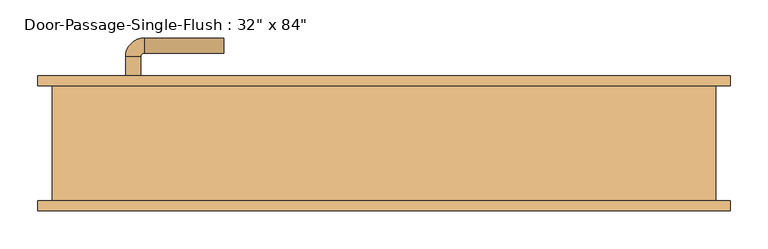
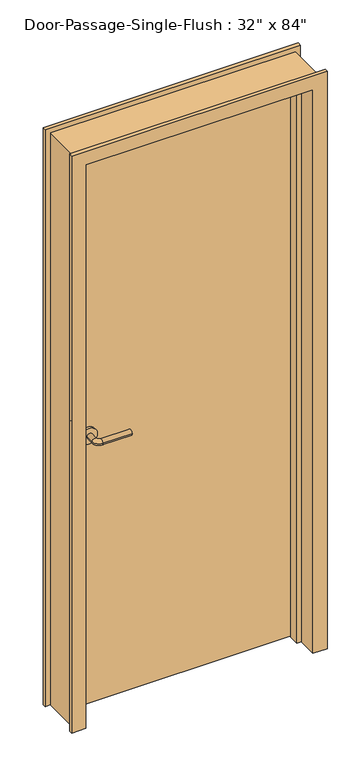
"""IFC4 building model written with IfcOpenShell, lengths in millimetres: door geometry."""

from ifc_helpers import new_model, si_unit, point, frame, frame_2d, origin, origin_with_axes, place, context, project, spatial, polyline, circle_curve, ellipse_curve, trimmed, segment, composite_curve, outline, extrude, faceted_brep, source, transform, mapped, element, save
from ifc_brep_helpers import plane_surface, cylinder_surface, revolved_surface, advanced_brep


def door_a08b6fcc(model_context):
    return source(origin(), model_context, "Body", "SolidModel", [
        advanced_brep(
        [(-341.390625, 23.75, 1016.0), (-321.390625, 23.75, 1016.0), (-321.390625, -6.25, 1016.0), (-341.390625, -6.25, 1016.0), (-316.390625, -11.25, 1016.0), (-316.390625, -31.25, 1016.0), (-211.390625, -31.25, 1016.0), (-211.390625, -11.25, 1016.0)],
        [
            (0, 1, circle_curve(frame((-331.390625, 23.75, 1016.0), z_axis=(0.0, 1.0, 0.0), x_axis=(1.0, 0.0, 0.0)), 10.0)),
            (1, 0, circle_curve(frame((-331.390625, 23.75, 1016.0), z_axis=(0.0, 1.0, 0.0), x_axis=(1.0, 0.0, 0.0)), 10.0)),
            (1, 2),
            (2, 3, circle_curve(frame((-331.390625, -6.25, 1016.0), z_axis=(0.0, 1.0, 0.0), x_axis=(1.0, 0.0, 0.0)), 10.0)),
            (3, 0),
            (3, 2, circle_curve(frame((-331.390625, -6.25, 1016.0), z_axis=(0.0, 1.0, 0.0), x_axis=(1.0, 0.0, 0.0)), 10.0)),
            (4, 5, circle_curve(frame((-316.390625, -21.25, 1016.0), z_axis=(-1.0, 0.0, 0.0), x_axis=(0.0, 1.0, 0.0)), 10.0)),
            (5, 3, circle_curve(frame((-316.390625, -6.25, 1016.0), z_axis=(0.0, 0.0, -1.0), x_axis=(-1.0, 0.0, 0.0)), 25.0)),
            (2, 4, circle_curve(frame((-316.390625, -6.25, 1016.0), z_axis=(0.0, 0.0, 1.0), x_axis=(-1.0, 0.0, 0.0)), 5.0)),
            (5, 4, circle_curve(frame((-316.390625, -21.25, 1016.0), z_axis=(-1.0, 0.0, 0.0), x_axis=(0.0, 1.0, 0.0)), 10.0)),
            (6, 7, circle_curve(frame((-211.390625, -21.25, 1016.0), z_axis=(1.0, 0.0, 0.0), x_axis=(0.0, 1.0, 0.0)), 10.0)),
            (7, 6, circle_curve(frame((-211.390625, -21.25, 1016.0), z_axis=(1.0, 0.0, 0.0), x_axis=(0.0, 1.0, 0.0)), 10.0)),
            (4, 7),
            (6, 5),
        ],
        [
            plane_surface(frame((-331.390625, 23.75, 1016.0), z_axis=(0.0, 1.0, 0.0), x_axis=(0.0, 0.0, 1.0))),
            cylinder_surface(frame((-331.390625, 23.75, 1016.0), z_axis=(0.0, 1.0, 0.0), x_axis=(1.0, 0.0, 0.0)), 10.0),
            revolved_surface(trimmed(ellipse_curve(frame((-331.390625, -6.25, 1016.0), z_axis=(0.0, -1.0, 0.0), x_axis=(1.0, 0.0, 0.0)), 10.0, 10.0), [point((-341.390625, -6.25, 1016.0))], [point((-321.390625, -6.25, 1016.0))], True, "CARTESIAN"), (-316.390625, -6.25, 1016.0), (0.0, 0.0, -1.0)),
            revolved_surface(trimmed(ellipse_curve(frame((-331.390625, -6.25, 1016.0), z_axis=(0.0, -1.0, 0.0), x_axis=(1.0, 0.0, 0.0)), 10.0, 10.0), [point((-321.390625, -6.25, 1016.0))], [point((-341.390625, -6.25, 1016.0))], True, "CARTESIAN"), (-316.390625, -6.25, 1016.0), (0.0, 0.0, -1.0)),
            plane_surface(frame((-211.390625, -21.25, 1016.0), z_axis=(1.0, 0.0, 0.0), x_axis=(0.0, 0.0, 1.0))),
            cylinder_surface(frame((-316.390625, -21.25, 1016.0), z_axis=(-1.0, 0.0, 0.0), x_axis=(0.0, 1.0, 0.0)), 10.0),
        ],
        [
            (0, [[1, 2]]),
            (1, [[3, 4, 5, -2]]),
            (1, [[-5, 6, -3, -1]]),
            (2, [[7, 8, -4, 9]]),
            (3, [[10, -9, -6, -8]]),
            (4, [[11, 12]]),
            (5, [[13, -11, 14, -7]]),
            (5, [[-14, -12, -13, -10]]),
        ],
    ),
        extrude(outline(composite_curve([segment(trimmed(circle_curve(frame_2d((1016.0, -333.890625)), 30.0), [point((1016.0, -363.890625))], [point((1016.0, -303.890625))], False, "CARTESIAN"), True, "CONTINUOUS"), segment(trimmed(circle_curve(frame_2d((1016.0, -333.890625)), 30.0), [point((1016.0, -303.890625))], [point((1016.0, -363.890625))], False, "CARTESIAN"), True, "CONTINUOUS")], self_intersect=False)), frame((0.0, 23.75, 0.0), z_axis=(0.0, 1.0, 0.0), x_axis=(0.0, 0.0, 1.0)), (0.0, 0.0, 1.0), 8.0),
        advanced_brep(
        [(-341.390625, 90.55, 1016.0), (-321.390625, 90.55, 1016.0), (-341.390625, 120.55, 1016.0), (-321.390625, 120.55, 1016.0), (-316.390625, 125.55, 1016.0), (-316.390625, 145.55, 1016.0), (-211.390625, 145.55, 1016.0), (-211.390625, 125.55, 1016.0)],
        [
            (0, 1, circle_curve(frame((-331.390625, 90.55, 1016.0), z_axis=(0.0, -1.0, 0.0), x_axis=(1.0, 0.0, 0.0)), 10.0)),
            (1, 0, circle_curve(frame((-331.390625, 90.55, 1016.0), z_axis=(0.0, -1.0, 0.0), x_axis=(1.0, 0.0, 0.0)), 10.0)),
            (0, 2),
            (2, 3, circle_curve(frame((-331.390625, 120.55, 1016.0), z_axis=(0.0, -1.0, 0.0), x_axis=(1.0, 0.0, 0.0)), 10.0)),
            (3, 1),
            (3, 2, circle_curve(frame((-331.390625, 120.55, 1016.0), z_axis=(0.0, -1.0, 0.0), x_axis=(1.0, 0.0, 0.0)), 10.0)),
            (4, 3, circle_curve(frame((-316.390625, 120.55, 1016.0), z_axis=(0.0, 0.0, 1.0), x_axis=(-1.0, 0.0, 0.0)), 5.0)),
            (2, 5, circle_curve(frame((-316.390625, 120.55, 1016.0), z_axis=(0.0, 0.0, -1.0), x_axis=(-1.0, 0.0, 0.0)), 25.0)),
            (5, 4, circle_curve(frame((-316.390625, 135.55, 1016.0), z_axis=(-1.0, 0.0, 0.0), x_axis=(0.0, -1.0, 0.0)), 10.0)),
            (4, 5, circle_curve(frame((-316.390625, 135.55, 1016.0), z_axis=(-1.0, 0.0, 0.0), x_axis=(0.0, -1.0, 0.0)), 10.0)),
            (6, 7, circle_curve(frame((-211.390625, 135.55, 1016.0), z_axis=(1.0, 0.0, 0.0), x_axis=(0.0, -1.0, 0.0)), 10.0)),
            (7, 6, circle_curve(frame((-211.390625, 135.55, 1016.0), z_axis=(1.0, 0.0, 0.0), x_axis=(0.0, -1.0, 0.0)), 10.0)),
            (5, 6),
            (7, 4),
        ],
        [
            plane_surface(frame((-331.390625, 90.55, 1016.0), z_axis=(0.0, -1.0, 0.0), x_axis=(0.0, 0.0, 1.0))),
            cylinder_surface(frame((-331.390625, 90.55, 1016.0), z_axis=(0.0, -1.0, 0.0), x_axis=(1.0, 0.0, 0.0)), 10.0),
            revolved_surface(trimmed(ellipse_curve(frame((-331.390625, 120.55, 1016.0), z_axis=(0.0, -1.0, 0.0), x_axis=(1.0, 0.0, 0.0)), 10.0, 10.0), [point((-341.390625, 120.55, 1016.0))], [point((-321.390625, 120.55, 1016.0))], True, "CARTESIAN"), (-316.390625, 120.55, 1016.0), (0.0, 0.0, -1.0)),
            revolved_surface(trimmed(ellipse_curve(frame((-331.390625, 120.55, 1016.0), z_axis=(0.0, -1.0, 0.0), x_axis=(1.0, 0.0, 0.0)), 10.0, 10.0), [point((-321.390625, 120.55, 1016.0))], [point((-341.390625, 120.55, 1016.0))], True, "CARTESIAN"), (-316.390625, 120.55, 1016.0), (0.0, 0.0, -1.0)),
            plane_surface(frame((-211.390625, 135.55, 1016.0), z_axis=(1.0, 0.0, 0.0), x_axis=(0.0, 0.0, 1.0))),
            cylinder_surface(frame((-316.390625, 135.55, 1016.0), z_axis=(-1.0, 0.0, 0.0), x_axis=(0.0, -1.0, 0.0)), 10.0),
        ],
        [
            (0, [[1, 2]]),
            (1, [[-1, 3, 4, 5]]),
            (1, [[-2, -5, 6, -3]]),
            (2, [[7, -4, 8, 9]]),
            (3, [[-8, -6, -7, 10]]),
            (4, [[11, 12]]),
            (5, [[-9, 13, -12, 14]]),
            (5, [[-10, -14, -11, -13]]),
        ],
    ),
        extrude(outline(composite_curve([segment(trimmed(circle_curve(frame_2d((1016.0, -333.890625)), 30.0), [point((1016.0, -363.890625))], [point((1016.0, -303.890625))], False, "CARTESIAN"), True, "CONTINUOUS"), segment(trimmed(circle_curve(frame_2d((1016.0, -333.890625)), 30.0), [point((1016.0, -303.890625))], [point((1016.0, -363.890625))], False, "CARTESIAN"), True, "CONTINUOUS")], self_intersect=False)), frame((0.0, 82.55, 0.0), z_axis=(0.0, 1.0, 0.0), x_axis=(0.0, 0.0, 1.0)), (0.0, 0.0, 1.0), 8.0),
        faceted_brep([(406.4, 95.25, 0.0), (457.2, 95.25, 0.0), (457.2, 82.55, 0.0), (438.15, 82.55, 0.0), (438.15, -69.85, 0.0), (457.2, -69.85, 0.0), (457.2, -82.55, 0.0), (406.4, -82.55, 0.0), (406.4, -11.1125, 0.0), (390.525, -11.1125, 0.0), (390.525, 26.9875, 0.0), (406.4, 26.9875, 0.0), (406.4, 95.25, 2133.6), (-406.4, 95.25, 2133.6), (-406.4, 95.25, 0.0), (-457.2, 95.25, 0.0), (-457.2, 95.25, 2184.4), (457.2, 95.25, 2184.4), (457.2, 82.55, 2184.4), (-457.2, 82.55, 2184.4), (-457.2, 82.55, 0.0), (-438.15, 82.55, 0.0), (-438.15, 82.55, 2165.35), (438.15, 82.55, 2165.35), (438.15, -69.85, 2165.35), (-438.15, -69.85, 2165.35), (-438.15, -69.85, 0.0), (-457.2, -69.85, 0.0), (-457.2, -69.85, 2184.4), (457.2, -69.85, 2184.4), (457.2, -82.55, 2184.4), (-457.2, -82.55, 2184.4), (-457.2, -82.55, 0.0), (-406.4, -82.55, 0.0), (-406.4, -82.55, 2133.6), (406.4, -82.55, 2133.6), (406.4, -11.1125, 2133.6), (-406.4, -11.1125, 2133.6), (-406.4, -11.1125, 0.0), (-390.525, -11.1125, 0.0), (-390.525, -11.1125, 2117.725), (390.525, -11.1125, 2117.725), (390.525, 26.9875, 2117.725), (-390.525, 26.9875, 2117.725), (-390.525, 26.9875, 0.0), (-406.4, 26.9875, 0.0), (-406.4, 26.9875, 2133.6), (406.4, 26.9875, 2133.6)], [[[0, 1, 2, 3, 4, 5, 6, 7, 8, 9, 10, 11]], [[1, 0, 12, 13, 14, 15, 16, 17]], [[2, 1, 17, 18]], [[3, 2, 18, 19, 20, 21, 22, 23]], [[4, 3, 23, 24]], [[5, 4, 24, 25, 26, 27, 28, 29]], [[6, 5, 29, 30]], [[7, 6, 30, 31, 32, 33, 34, 35]], [[8, 7, 35, 36]], [[9, 8, 36, 37, 38, 39, 40, 41]], [[10, 9, 41, 42]], [[11, 10, 42, 43, 44, 45, 46, 47]], [[0, 11, 47, 12]], [[18, 17, 16, 19]], [[24, 23, 22, 25]], [[30, 29, 28, 31]], [[36, 35, 34, 37]], [[42, 41, 40, 43]], [[12, 47, 46, 13]], [[14, 45, 44, 39, 38, 33, 32, 27, 26, 21, 20, 15]], [[19, 16, 15, 20]], [[25, 22, 21, 26]], [[31, 28, 27, 32]], [[37, 34, 33, 38]], [[43, 40, 39, 44]], [[13, 46, 45, 14]]]),
        extrude(outline(polyline([(406.4, 31.75), (-406.4, 31.75), (-406.4, 82.55), (406.4, 82.55), (406.4, 31.75)])), origin_with_axes(), (0.0, 0.0, 1.0), 2133.6),
    ])


if __name__ == "__main__":
    model = new_model("IFC4")
    model_context = context("Model", 3, world=origin())
    ifc_project = project(units=[si_unit("LENGTHUNIT", "METRE", prefix="MILLI")], contexts=[model_context])
    site = spatial("IfcSite", under=ifc_project)
    building = spatial("IfcBuilding", under=site)
    placement = place(None, origin())
    door_shape = door_a08b6fcc(model_context)
    element("IfcDoor", 1, ObjectType="Door-Passage-Single-Flush : 32\" x 84\"", at=placement, inside=building, context=model_context, shape_type="MappedRepresentation", body=[
        mapped(door_shape, transform((0.0, 0.0, 0.0), x_axis=(1.0, 0.0, 0.0), y_axis=(0.0, 1.0, 0.0), z_axis=(0.0, 0.0, 1.0))),
    ])
    save(model, "model.ifc")

# Revit data of these elements
# Type "Door-Passage-Single-Flush : 32\" x 84\""
#   Type Mark = "10"
#   Assembly Code = "C1020"
#   Analytic Construction = "Wooden"
#   Thickness = 0' - 2"
#   Thermal Resistance (R) = 2.5876 (h·ft²·°F)/BTU
#   Swing Angle [instance default] = 90.00°
#   Strike Height = 3' - 4"
#   Rough Width [instance default] = 3' - 0"
#   Rough Height [instance default] = 7' - 4"
#   Masonry Inset [instance default] = 0' - 1"
#   Masonry Frame Depth = 0' - 5 3/4"
#   MF Opening Width [instance default] = 0' - 4"
#   MF Opening Height [instance default] = 0' - 4"
#   Inset Calculate [instance default] = 0' - 4"
#   Heat Transfer Coefficient (U) = 0.3865 BTU/(h·ft²·°F)
#   Height = 7' - 0"
#   Width = 2' - 8"
#   Masonry Frame [instance default] = yes
#   Dry Wall Frame [instance default] = no
#   Panel Material = Wood - Birch
#   Door Handle Material = Aluminum
#   Frame Material = Door - Frame
#   Visual Light Transmittance = 0
#   Solar Heat Gain Coefficient = 0
#   Function = (empty or 0)
#   Wall Closure = (empty or 0)
# Element 1 (IfcDoor, "Door-Passage-Single-Flush : 32\" x 84\"")
#   Rough Width = 2' - 10 1/2"
#   Rough Height = 7' - 1 1/4"
#   MF Opening Width = 0' - 2 1/2"
#   MF Opening Height = 0' - 1 1/4"
#   Inset Calculate = 0' - 3"
#   Masonry Frame = no
#   Dry Wall Frame = yes
#   Materials on its faces: "Door - Frame", "Aluminum", "Wood - Birch"
# Materials
#   "Wood - Birch": class "Unassigned", colour RGB 224 178 126, transparency 0
#   "Aluminum": class "Metal", colour RGB 244 244 244, transparency 0, Description = "Aluminum 6061", Cost = 0
#   "Door - Frame": class "Unassigned", colour RGB 118 70 51, transparency 0
